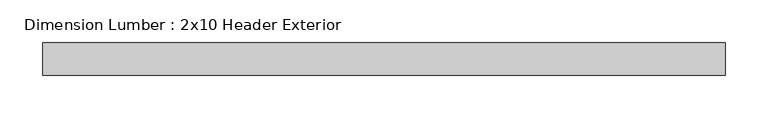
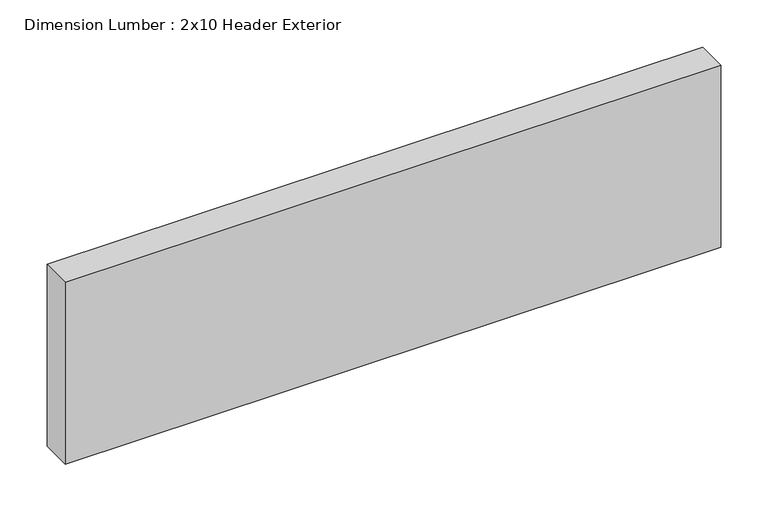
"""IFC4 building model written with IfcOpenShell, lengths in millimetres: beam geometry, Dimension Lumber : 2x10 Header Exterior."""

from ifc_helpers import new_model, si_unit, frame, origin, place, context, project, spatial, polyline, outline, extrude, source, transform, mapped, element, save


def dimension_lumber_2x10_header_exterior_c5c52a49(model_context):
    return source(origin(), model_context, "Body", "SweptSolid", [
        extrude(outline(polyline([(468.709375, 19.05), (468.709375, -19.05), (-331.390625, -19.05), (-331.390625, 19.05), (468.709375, 19.05)])), frame((0.0, 0.0, -117.475), z_axis=(0.0, 0.0, 1.0), x_axis=(1.0, 0.0, 0.0)), (0.0, 0.0, 1.0), 234.95),
    ])


if __name__ == "__main__":
    model = new_model("IFC4")
    model_context = context("Model", 3, world=origin())
    ifc_project = project(units=[si_unit("LENGTHUNIT", "METRE", prefix="MILLI")], contexts=[model_context])
    site = spatial("IfcSite", under=ifc_project)
    building = spatial("IfcBuilding", under=site)
    placement = place(None, origin())
    dimension_lumber_2x10_header_exterior_shape = dimension_lumber_2x10_header_exterior_c5c52a49(model_context)
    element("IfcBeam", 1, ObjectType="Dimension Lumber : 2x10 Header Exterior", at=placement, inside=building, context=model_context, shape_type="MappedRepresentation", body=[
        mapped(dimension_lumber_2x10_header_exterior_shape, transform((0.0, 0.0, 0.0), x_axis=(1.0, 0.0, 0.0), y_axis=(0.0, 1.0, 0.0), z_axis=(0.0, 0.0, 1.0))),
    ])
    save(model, "model.ifc")

# Revit data of these elements
# Type "Dimension Lumber : 2x10 Header Exterior"
#   Assembly Code = "B10"
#   A = 0.0963889 SF
#   Length [instance default] = 5' - 0"
#   b = 0' - 1 1/2"
#   d = 0' - 9 1/4"
#   Structural Material [instance default] = Softwood, Lumber
# Element 1 (IfcBeam, "Dimension Lumber : 2x10 Header Exterior")
#   Structural Material = Douglas Fir #2
#   Materials on its faces: "Douglas Fir #2"
# Materials
#   "Softwood, Lumber": class "Wood", colour RGB 223 192 134, transparency 0, Description = "Pinus Echinata", Cost = 0
#   "Douglas Fir #2": class "Wood", colour RGB 223 192 134, transparency 0, Description = "Pinus Echinata", Cost = 0
